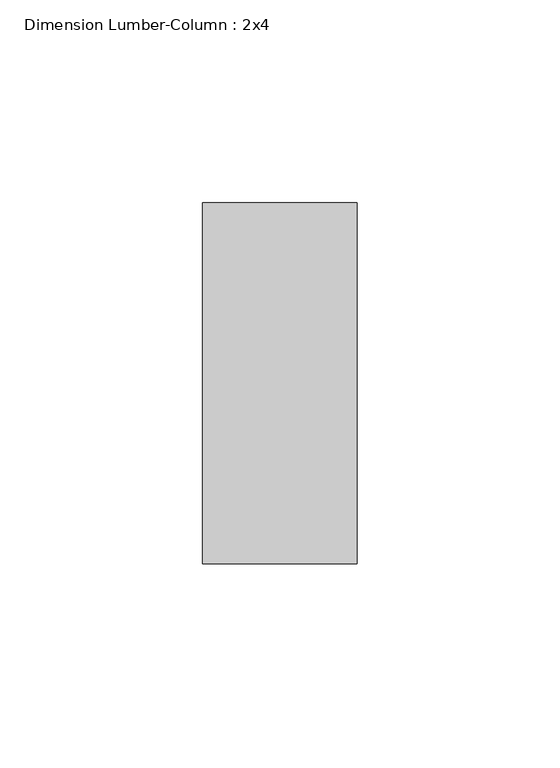
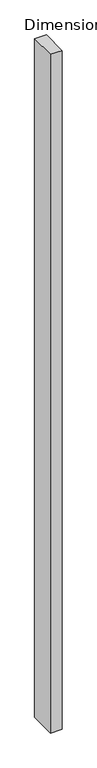
"""IFC4 building model written with IfcOpenShell, lengths in millimetres: column geometry, Dimension Lumber-Column : 2x4."""

from ifc_helpers import new_model, si_unit, frame, origin, place, context, project, spatial, polyline, outline, extrude, source, transform, mapped, element, save


def dimension_lumber_column_2x4_1c0ee4a5(model_context):
    return source(origin(), model_context, "Body", "SweptSolid", [
        extrude(outline(polyline([(19.05, -44.45), (-19.05, -44.45), (-19.05, 44.45), (19.05, 44.45), (19.05, -44.45)])), frame((0.0, 0.0, 56.35625), z_axis=(0.0, 0.0, 1.0), x_axis=(1.0, 0.0, 0.0)), (0.0, 0.0, 1.0), 2331.24375),
    ])


if __name__ == "__main__":
    model = new_model("IFC4")
    model_context = context("Model", 3, world=origin())
    ifc_project = project(units=[si_unit("LENGTHUNIT", "METRE", prefix="MILLI")], contexts=[model_context])
    site = spatial("IfcSite", under=ifc_project)
    building = spatial("IfcBuilding", under=site)
    placement = place(None, origin())
    dimension_lumber_column_2x4_shape = dimension_lumber_column_2x4_1c0ee4a5(model_context)
    element("IfcColumn", 1, ObjectType="Dimension Lumber-Column : 2x4", at=placement, inside=building, context=model_context, shape_type="MappedRepresentation", body=[
        mapped(dimension_lumber_column_2x4_shape, transform((0.0, 0.0, 0.0), x_axis=(1.0, 0.0, 0.0), y_axis=(0.0, 1.0, 0.0), z_axis=(0.0, 0.0, 1.0))),
    ])
    save(model, "model.ifc")

# Revit data of these elements
# Type "Dimension Lumber-Column : 2x4"
#   Int Type = "Interior"
#   Assembly Code = "B10"
#   Cost = 8.05
#   A = 0.0364583 SF
#   b = 0' - 1 1/2"
#   d = 0' - 3 1/2"
#   Structural Material [instance default] = Softwood, Lumber
# Element 1 (IfcColumn, "Dimension Lumber-Column : 2x4")
#   Structural Material = Douglas Fir #2
#   Materials on its faces: "Douglas Fir #2"
# Materials
#   "Softwood, Lumber": class "Wood", colour RGB 223 192 134, transparency 0, Description = "Pinus Echinata", Cost = 0
#   "Douglas Fir #2": class "Wood", colour RGB 223 192 134, transparency 0, Description = "Pinus Echinata", Cost = 0
